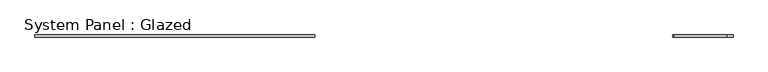
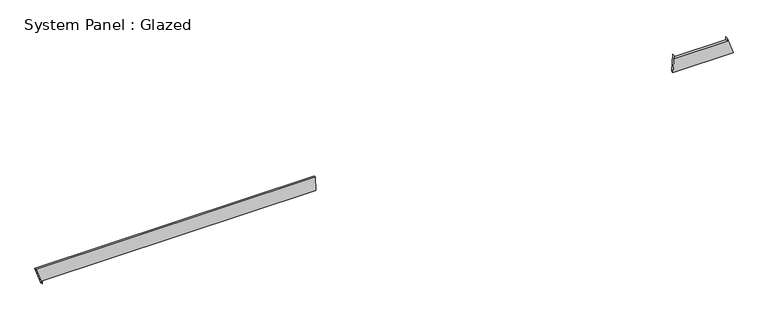
"""IFC4 building model written with IfcOpenShell, lengths in millimetres: plate geometry, System Panel : Glazed."""

from ifc_helpers import new_model, si_unit, frame, origin, place, context, project, spatial, polyline, outline, extrude, source, transform, mapped, element, save


def system_panel_glazed_0701c0ee(model_context):
    return source(origin(), model_context, "Body", "SweptSolid", [
        extrude(outline(polyline([(35.3553391, 3330.5569074), (35.3553391, 4027.9323725), (235.7126054, 3959.1507422), (200.3572664, 3959.151181), (200.349652, 3345.7415652), (235.7049911, 3345.7411263), (35.3553391, 3330.5569074)])), frame((0.0, -49.5, 0.0), z_axis=(0.0, 1.0, 0.0), x_axis=(0.0, 0.0, 1.0)), (0.0, 0.0, 1.0), 25.0),
        extrude(outline(polyline([(0.0, -3958.9104535), (35.3553391, -3958.9104535), (35.3553391, -798.4718208), (200.2981725, -801.4418115), (200.2581216, -4027.9323725), (0.0, -3958.9104535)])), frame((0.0, -49.5, 0.0), z_axis=(0.0, 1.0, 0.0), x_axis=(0.0, 0.0, 1.0)), (0.0, 0.0, 1.0), 25.0),
    ])


if __name__ == "__main__":
    model = new_model("IFC4")
    model_context = context("Model", 3, world=origin())
    ifc_project = project(units=[si_unit("LENGTHUNIT", "METRE", prefix="MILLI")], contexts=[model_context])
    site = spatial("IfcSite", under=ifc_project)
    building = spatial("IfcBuilding", under=site)
    placement = place(None, origin())
    system_panel_glazed_shape = system_panel_glazed_0701c0ee(model_context)
    element("IfcPlate", 1, ObjectType="System Panel : Glazed", at=placement, inside=building, context=model_context, shape_type="MappedRepresentation", body=[
        mapped(system_panel_glazed_shape, transform((0.0, 0.0, 0.0), x_axis=(1.0, 0.0, 0.0), y_axis=(0.0, 1.0, 0.0), z_axis=(0.0, 0.0, 1.0))),
    ])
    save(model, "model.ifc")

# Revit data of these elements
# Element 1 (IfcPlate, "System Panel : Glazed")
#   Materials on its faces: "Glass"
# Materials
#   "Glass": class "Glass", colour RGB 218 227 224, transparency 0.85, Description = "Soda Lime Glass", Cost = 0
